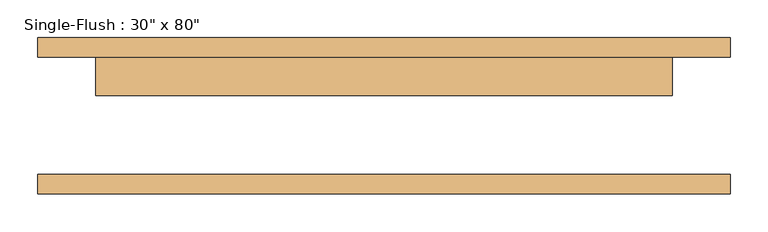
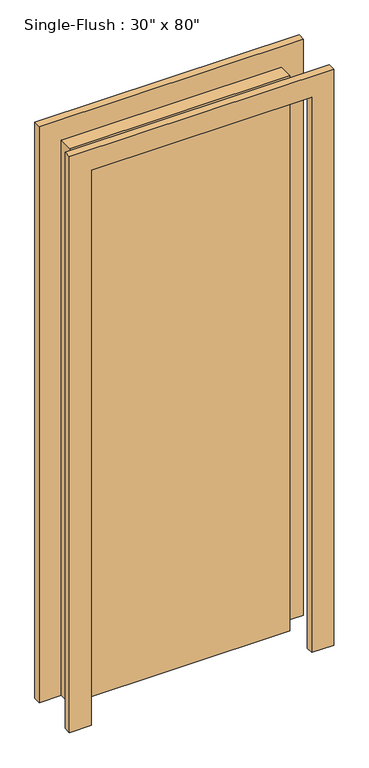
"""IFC4 building model written with IfcOpenShell, lengths in millimetres: door geometry."""

import ifcopenshell
import ifcopenshell.guid

model = None  # the IFC model being written
_history = None  # IfcOwnerHistory: only IFC2X3 demands one
_inside = {}  # id of a spatial element -> (the spatial element, [elements in it])
_under = {}  # id of a project, library or spatial element -> (it, [spatial elements below it])
_declared = {}  # id of a project -> (the project, [libraries it declares])
_typed = {}  # id of a type object -> (the type object, [elements of that type])
_made_of = {}  # id of a material, layer set ... -> (it, [elements and type objects made of it])


def new_model(schema):
    """Start an empty IFC model of exactly this schema.

    Asked for "IFC4X3", IfcOpenShell would pick the latest addendum, in which some entities
    have other attributes; the version numbers below select the first issue.
    IFC2X3 requires an IfcOwnerHistory on every rooted entity: one is made here for all.
    """
    global model, _history
    if schema == "IFC4X3":
        model = ifcopenshell.file(schema_version=(4, 3, 0, 0))
    else:
        model = ifcopenshell.file(schema=schema)
    _inside.clear()
    _under.clear()
    _declared.clear()
    _typed.clear()
    _made_of.clear()
    _history = None
    if model.schema == "IFC2X3":
        org = make("IfcOrganization", Name="unknown")
        user = make(
            "IfcPersonAndOrganization",
            ThePerson=make("IfcPerson", FamilyName="unknown"),
            TheOrganization=org,
        )
        app = make(
            "IfcApplication",
            ApplicationDeveloper=org,
            Version="unknown",
            ApplicationFullName="unknown",
            ApplicationIdentifier="unknown",
        )
        _history = make(
            "IfcOwnerHistory",
            OwningUser=user,
            OwningApplication=app,
            ChangeAction="ADDED",
            CreationDate=0,
        )
    return model


def make(cls, **values):
    """One entity of the class cls with the attributes given. An attribute that is None is left unset."""
    return model.create_entity(
        cls, **{name: value for name, value in values.items() if value is not None}
    )


def rooted(cls, **values):
    """An entity with a GlobalId (a new one), such as an element, a storey or a relation."""
    return make(cls, GlobalId=ifcopenshell.guid.new(), OwnerHistory=_history, **values)


def si_unit(unit_type, name, prefix=None):
    """IfcSIUnit, for example si_unit("LENGTHUNIT", "METRE", prefix="MILLI")."""
    return make("IfcSIUnit", UnitType=unit_type, Prefix=prefix, Name=name)


def assignment(units):
    """IfcUnitAssignment: the units of a project."""
    return None if units is None else make("IfcUnitAssignment", Units=units)


def point(xyz):
    """IfcCartesianPoint."""
    return None if xyz is None else make("IfcCartesianPoint", Coordinates=xyz)


def direction(xyz):
    """IfcDirection."""
    return None if xyz is None else make("IfcDirection", DirectionRatios=xyz)


def frame(location, z_axis=None, x_axis=None):
    """IfcAxis2Placement3D, a coordinate frame: its origin and axes. An axis left out is left unset."""
    return make(
        "IfcAxis2Placement3D",
        Location=point(location),
        Axis=direction(z_axis),
        RefDirection=direction(x_axis),
    )


def origin():
    """The frame at (0, 0, 0) with its axes left unset."""
    return frame((0.0, 0.0, 0.0))


def origin_with_axes():
    """The frame at (0, 0, 0) with the z axis (0, 0, 1) and the x axis (1, 0, 0) written out."""
    return frame((0.0, 0.0, 0.0), z_axis=(0.0, 0.0, 1.0), x_axis=(1.0, 0.0, 0.0))


def place(relative_to, where):
    """IfcLocalPlacement: puts the frame where relative to a parent placement (None: the world)."""
    return make(
        "IfcLocalPlacement", PlacementRelTo=relative_to, RelativePlacement=where
    )


def context(
    kind, dimensions, precision=None, world=None, true_north=None, identifier=None
):
    """IfcGeometricRepresentationContext, for example the 3D "Model" context."""
    return make(
        "IfcGeometricRepresentationContext",
        ContextIdentifier=identifier,
        ContextType=kind,
        CoordinateSpaceDimension=dimensions,
        Precision=precision,
        WorldCoordinateSystem=world,
        TrueNorth=true_north,
    )


def project(units=None, contexts=None):
    """IfcProject with its units and contexts."""
    return rooted(
        "IfcProject",
        Name="project",
        RepresentationContexts=contexts,
        UnitsInContext=assignment(units),
    )


def spatial(cls, under=None, at=None, **own):
    """A site, building, storey or space (cls), placed at a placement, below another one or the project."""
    s = rooted(cls, ObjectPlacement=at, **own)
    if under is not None:
        _under.setdefault(under.id(), (under, []))[1].append(s)
    return s


def polyline(points):
    """IfcPolyline through the points."""
    return make("IfcPolyline", Points=[point(p) for p in points])


def outline(outer, holes=None, kind="AREA"):
    """IfcArbitraryClosedProfileDef: a profile drawn as a closed curve; with holes, ...WithVoids."""
    if holes is None:
        return make("IfcArbitraryClosedProfileDef", ProfileType=kind, OuterCurve=outer)
    return make(
        "IfcArbitraryProfileDefWithVoids",
        ProfileType=kind,
        OuterCurve=outer,
        InnerCurves=holes,
    )


def extrude(swept, where, along, depth):
    """IfcExtrudedAreaSolid: the profile swept, set in the frame where, extruded along a direction by depth."""
    return make(
        "IfcExtrudedAreaSolid",
        SweptArea=swept,
        Position=where,
        ExtrudedDirection=direction(along),
        Depth=depth,
    )


def shape(context_of_items, identifier, shape_type, items):
    """IfcShapeRepresentation: the items that make up one representation, for example the "Body"."""
    return make(
        "IfcShapeRepresentation",
        ContextOfItems=context_of_items,
        RepresentationIdentifier=identifier,
        RepresentationType=shape_type,
        Items=items,
    )


def source(mapping_origin, context_of_items, identifier, shape_type, items):
    """IfcRepresentationMap: a shape defined once, which mapped items show again and again."""
    return make(
        "IfcRepresentationMap",
        MappingOrigin=mapping_origin,
        MappedRepresentation=shape(context_of_items, identifier, shape_type, items),
    )


def transform(
    local_origin,
    x_axis=None,
    y_axis=None,
    z_axis=None,
    scale=None,
    scale2=None,
    scale3=None,
    uniform=True,
):
    """IfcCartesianTransformationOperator3D, or its non-uniform kind. x_axis, y_axis, z_axis: its Axis1, 2, 3."""
    if uniform:
        return make(
            "IfcCartesianTransformationOperator3D",
            Axis1=direction(x_axis),
            Axis2=direction(y_axis),
            LocalOrigin=point(local_origin),
            Scale=scale,
            Axis3=direction(z_axis),
        )
    return make(
        "IfcCartesianTransformationOperator3DnonUniform",
        Axis1=direction(x_axis),
        Axis2=direction(y_axis),
        LocalOrigin=point(local_origin),
        Scale=scale,
        Axis3=direction(z_axis),
        Scale2=scale2,
        Scale3=scale3,
    )


def mapped(mapping_source, mapping_target):
    """IfcMappedItem: shows the shape of a source again, moved by a transform."""
    return make(
        "IfcMappedItem", MappingSource=mapping_source, MappingTarget=mapping_target
    )


def made_of(thing, what):
    """Note that an element or type object is made of a material, layer set ...; save() writes the relation."""
    if what is not None:
        _made_of.setdefault(what.id(), (what, []))[1].append(thing)
    return thing


def element(
    cls,
    number,
    at=None,
    inside=None,
    cuts=None,
    type_object=None,
    material=None,
    context=None,
    identifier="Body",
    shape_type=None,
    held_by="IfcProductDefinitionShape",
    body=None,
    shapes=None,
    **own,
):
    """One element of the class cls, such as IfcWall. Its Tag is "e" and its number.

    at: its placement. inside: the storey or other place that contains it. cuts: it is an
    opening in that element (IfcRelVoidsElement). A single representation is given by context,
    identifier, shape_type and body (its items); several are given by shapes. held_by: the class
    of the entity that holds the representations. save() writes the other relations.
    """
    e = rooted(cls, Tag="e%d" % number, ObjectPlacement=at, **own)
    if body is not None:
        shapes = [shape(context, identifier, shape_type, body)]
    if shapes is not None:
        e.Representation = make(held_by, Representations=shapes)
    if inside is not None:
        _inside.setdefault(inside.id(), (inside, []))[1].append(e)
    if cuts is not None:
        rooted(
            "IfcRelVoidsElement", RelatingBuildingElement=cuts, RelatedOpeningElement=e
        )
    if type_object is not None:
        _typed.setdefault(type_object.id(), (type_object, []))[1].append(e)
    return made_of(e, material)


def aggregate(whole, parts):
    """IfcRelAggregates: a whole, such as a stair, and the parts it consists of."""
    return rooted("IfcRelAggregates", RelatingObject=whole, RelatedObjects=parts)


def save(model, path):
    """Write the relations noted so far, then the file.

    IfcRelAggregates (storeys below a building ...), IfcRelContainedInSpatialStructure (elements
    in a storey), IfcRelDefinesByType, IfcRelAssociatesMaterial and IfcRelDeclares: one each for
    every whole, place, type object, material and project.
    """
    for whole, parts in _under.values():
        aggregate(whole, parts)
    for where, things in _inside.values():
        rooted(
            "IfcRelContainedInSpatialStructure",
            RelatedElements=things,
            RelatingStructure=where,
        )
    for kind, things in _typed.values():
        rooted("IfcRelDefinesByType", RelatedObjects=things, RelatingType=kind)
    for what, things in _made_of.values():
        rooted("IfcRelAssociatesMaterial", RelatedObjects=things, RelatingMaterial=what)
    for by, libraries in _declared.values():
        rooted("IfcRelDeclares", RelatingContext=by, RelatedDefinitions=libraries)
    model.write(path)


def door_a57ad9fa(model_context):
    return source(origin(), model_context, "Body", "SweptSolid", [
        extrude(outline(polyline([(2108.2, -457.2), (0.0, -457.2), (0.0, -381.0), (2032.0, -381.0), (2032.0, 381.0), (0.0, 381.0), (0.0, 457.2), (2108.2, 457.2), (2108.2, -457.2)])), frame((0.0, 77.7875, 0.0), z_axis=(0.0, 1.0, 0.0), x_axis=(0.0, 0.0, 1.0)), (0.0, 0.0, 1.0), 25.4),
        extrude(outline(polyline([(2108.2, 457.2), (2108.2, -457.2), (0.0, -457.2), (0.0, -381.0), (2032.0, -381.0), (2032.0, 381.0), (0.0, 381.0), (0.0, 457.2), (2108.2, 457.2)])), frame((0.0, -103.1875, 0.0), z_axis=(0.0, 1.0, 0.0), x_axis=(0.0, 0.0, 1.0)), (0.0, 0.0, 1.0), 25.4),
        extrude(outline(polyline([(381.0, 26.9875), (-381.0, 26.9875), (-381.0, 77.7875), (381.0, 77.7875), (381.0, 26.9875)])), origin_with_axes(), (0.0, 0.0, 1.0), 2032.0),
    ])


if __name__ == "__main__":
    model = new_model("IFC4")
    model_context = context("Model", 3, world=origin())
    ifc_project = project(units=[si_unit("LENGTHUNIT", "METRE", prefix="MILLI")], contexts=[model_context])
    site = spatial("IfcSite", under=ifc_project)
    building = spatial("IfcBuilding", under=site)
    placement = place(None, origin())
    door_shape = door_a57ad9fa(model_context)
    element("IfcDoor", 1, ObjectType="Single-Flush : 30\" x 80\"", at=placement, inside=building, context=model_context, shape_type="MappedRepresentation", body=[
        mapped(door_shape, transform((0.0, 0.0, 0.0), x_axis=(1.0, 0.0, 0.0), y_axis=(0.0, 1.0, 0.0), z_axis=(0.0, 0.0, 1.0))),
    ])
    save(model, "model.ifc")

# Revit data of these elements
# Project information
#   Project Issue Date = "Issue Date"
#   Project Status = "Project Status"
#   Client Name = "Owner"
#   Project Address = "Enter address here"
#   Project Name = "Project Name"
#   Project Number = "Project Number"
# Type "Single-Flush : 30\" x 80\""
#   Type Mark = "5"
#   Construction Type Id = "MDOOR"
#   Assembly Code = "C1020"
#   Analytic Construction = "Metal"
#   Thickness = 0' - 2"
#   Heat Transfer Coefficient (U) = 3.7021 W/(m²·K)
#   Height = 6' - 8"
#   Trim Projection Ext = 0' - 1"
#   Trim Projection Int = 0' - 1"
#   Trim Width = 0' - 3"
#   Width = 2' - 6"
#   Door Material = Door - Panel
#   Frame Material = Door - Frame
#   Visual Light Transmittance = 0
#   Solar Heat Gain Coefficient = 0
#   Function = (empty or 0)
#   Wall Closure = (empty or 0)
# Element 1 (IfcDoor, "Single-Flush : 30\" x 80\"")
#   Materials on its faces: "Door - Frame", "Door - Panel"
# Materials
#   "Door - Panel": class "Wood", colour RGB 210 159 95, transparency 0, Cost = 0
#   "Door - Frame": class "Miscellaneous", colour RGB 118 70 51, transparency 0, Cost = 0
